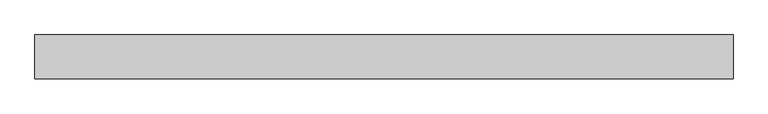
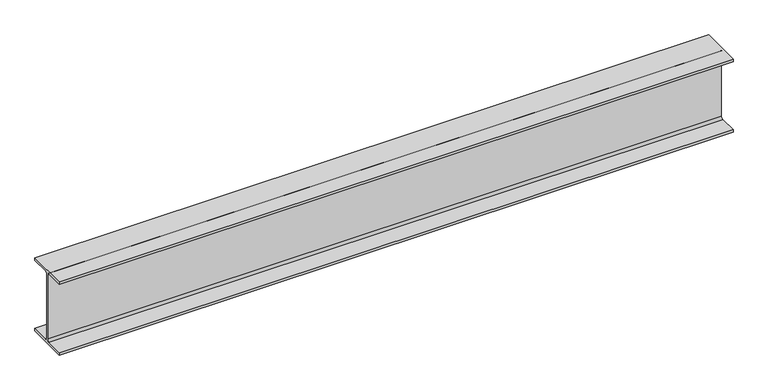
"""IFC4 building model written with IfcOpenShell, lengths in millimetres: beam geometry, Old_Steel Beam_H-KSD3502 : H_SB_ASB_H-250×125x6x9."""

from ifc_helpers import new_model, si_unit, point, frame, frame_2d, origin, place, context, project, spatial, polyline, circle_curve, trimmed, segment, composite_curve, outline, extrude, source, transform, mapped, element, save


def beam_b5d638d0(model_context):
    return source(origin(), model_context, "Body", "SweptSolid", [
        extrude(outline(composite_curve([segment(polyline([(82.5, -141.5), (82.5, -151.7), (-82.5, -151.7), (-82.5, -141.5), (-11.9, -141.5)]), True, "CONTINUOUS"), segment(trimmed(circle_curve(frame_2d((-11.9, -132.6)), 8.9), [point((-11.9, -141.5))], [point((-3.0, -132.6))], True, "CARTESIAN"), True, "CONTINUOUS"), segment(polyline([(-3.0, -132.6), (-3.0, 132.6)]), True, "CONTINUOUS"), segment(trimmed(circle_curve(frame_2d((-11.9, 132.6)), 8.9), [point((-3.0, 132.6))], [point((-11.9, 141.5))], True, "CARTESIAN"), True, "CONTINUOUS"), segment(polyline([(-11.9, 141.5), (-82.5, 141.5), (-82.5, 151.7), (82.5, 151.7), (82.5, 141.5), (11.9, 141.5)]), True, "CONTINUOUS"), segment(trimmed(circle_curve(frame_2d((11.9, 132.6)), 8.9), [point((11.9, 141.5))], [point((3.0, 132.6))], True, "CARTESIAN"), True, "CONTINUOUS"), segment(polyline([(3.0, 132.6), (3.0, -132.6)]), True, "CONTINUOUS"), segment(trimmed(circle_curve(frame_2d((11.9, -132.6)), 8.9), [point((3.0, -132.6))], [point((11.9, -141.5))], True, "CARTESIAN"), True, "CONTINUOUS"), segment(polyline([(11.9, -141.5), (82.5, -141.5)]), True, "CONTINUOUS")], self_intersect=False)), frame((-1387.3, 0.0, 0.0), z_axis=(1.0, 0.0, 0.0), x_axis=(0.0, 1.0, 0.0)), (0.0, 0.0, 1.0), 2636.6),
    ])


if __name__ == "__main__":
    model = new_model("IFC4")
    model_context = context("Model", 3, world=origin())
    ifc_project = project(units=[si_unit("LENGTHUNIT", "METRE", prefix="MILLI")], contexts=[model_context])
    site = spatial("IfcSite", under=ifc_project)
    building = spatial("IfcBuilding", under=site)
    placement = place(None, origin())
    beam_shape = beam_b5d638d0(model_context)
    element("IfcBeam", 1, ObjectType="Old_Steel Beam_H-KSD3502 : H_SB_ASB_H-250×125x6x9", at=placement, inside=building, context=model_context, shape_type="MappedRepresentation", body=[
        mapped(beam_shape, transform((0.0, 0.0, 0.0), x_axis=(1.0, 0.0, 0.0), y_axis=(0.0, 1.0, 0.0), z_axis=(0.0, 0.0, 1.0))),
    ])
    save(model, "model.ifc")

# Revit data of these elements
# Type "Old_Steel Beam_H-KSD3502 : H_SB_ASB_H-250×125x6x9"
#   Width = 12.5 cm
#   Web Thickness = 0.6 cm
#   Web Fillet = 1.2 cm
#   Warping Constant = 42539.8 cm⁶
#   Torsional Moment of Inertia = 7.8102 cm⁴
#   Torsional Modulus = 1.0 cm³
#   Section Area = 37.66 cm²
#   Plastic Modulus weak axis = 73.1 cm³
#   Plastic Modulus strong axis = 366.0 cm³
#   Perimeter = 0.97 m²/m
#   Nominal Weight = 29.60 kgf/m
#   Moment of Inertia weak axis = 294.00 cm⁴
#   Moment of Inertia strong axis = 4050.00 cm⁴
#   Height = 25.0 cm
#   Flange Thickness = 0.9 cm
#   Elastic Modulus weak axis = 47.0 cm³
#   Elastic Modulus strong axis = 324.0 cm³
#   Centroid Vertical = 12.5 cm
#   Centroid Horizontal = 6.25 cm
#   Length [instance default] = 1.5240 m
#   Structural Material [instance default] = Steel, 45-345
#   Assembly Code = ""
# Element 1 (IfcBeam, "Old_Steel Beam_H-KSD3502 : H_SB_ASB_H-250×125x6x9")
#   Structural Material = none
# Materials
#   "Steel, 45-345": class "Metal", colour RGB 189 187 185, transparency 0, Description = "Steel 345 MPa", Cost = 0
